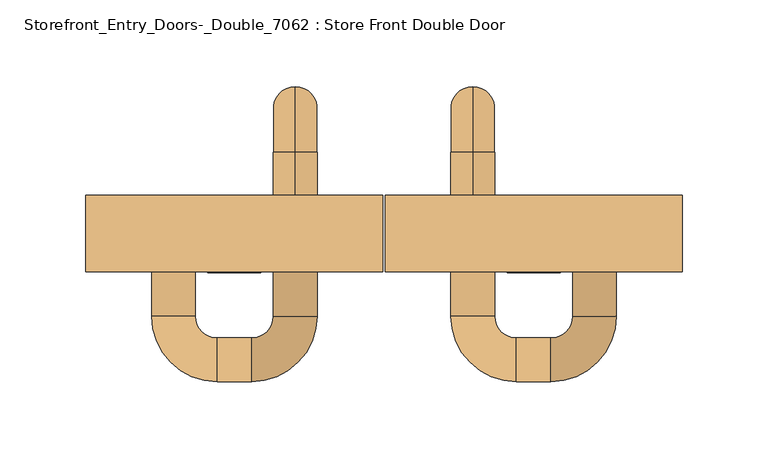
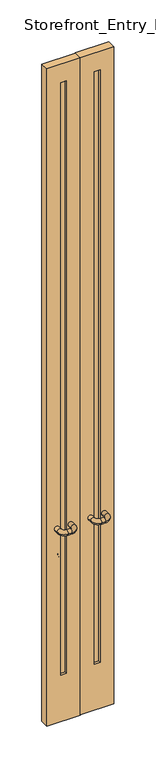
"""IFC4 building model written with IfcOpenShell, lengths in millimetres: door geometry, Storefront_Entry_Doors-_Double_7062 : Store Front Double Door."""

import ifcopenshell
import ifcopenshell.guid

model = None  # the IFC model being written
_history = None  # IfcOwnerHistory: only IFC2X3 demands one
_inside = {}  # id of a spatial element -> (the spatial element, [elements in it])
_under = {}  # id of a project, library or spatial element -> (it, [spatial elements below it])
_declared = {}  # id of a project -> (the project, [libraries it declares])
_typed = {}  # id of a type object -> (the type object, [elements of that type])
_made_of = {}  # id of a material, layer set ... -> (it, [elements and type objects made of it])


def new_model(schema):
    """Start an empty IFC model of exactly this schema.

    Asked for "IFC4X3", IfcOpenShell would pick the latest addendum, in which some entities
    have other attributes; the version numbers below select the first issue.
    IFC2X3 requires an IfcOwnerHistory on every rooted entity: one is made here for all.
    """
    global model, _history
    if schema == "IFC4X3":
        model = ifcopenshell.file(schema_version=(4, 3, 0, 0))
    else:
        model = ifcopenshell.file(schema=schema)
    _inside.clear()
    _under.clear()
    _declared.clear()
    _typed.clear()
    _made_of.clear()
    _history = None
    if model.schema == "IFC2X3":
        org = make("IfcOrganization", Name="unknown")
        user = make(
            "IfcPersonAndOrganization",
            ThePerson=make("IfcPerson", FamilyName="unknown"),
            TheOrganization=org,
        )
        app = make(
            "IfcApplication",
            ApplicationDeveloper=org,
            Version="unknown",
            ApplicationFullName="unknown",
            ApplicationIdentifier="unknown",
        )
        _history = make(
            "IfcOwnerHistory",
            OwningUser=user,
            OwningApplication=app,
            ChangeAction="ADDED",
            CreationDate=0,
        )
    return model


def make(cls, **values):
    """One entity of the class cls with the attributes given. An attribute that is None is left unset."""
    return model.create_entity(
        cls, **{name: value for name, value in values.items() if value is not None}
    )


def rooted(cls, **values):
    """An entity with a GlobalId (a new one), such as an element, a storey or a relation."""
    return make(cls, GlobalId=ifcopenshell.guid.new(), OwnerHistory=_history, **values)


def si_unit(unit_type, name, prefix=None):
    """IfcSIUnit, for example si_unit("LENGTHUNIT", "METRE", prefix="MILLI")."""
    return make("IfcSIUnit", UnitType=unit_type, Prefix=prefix, Name=name)


def assignment(units):
    """IfcUnitAssignment: the units of a project."""
    return None if units is None else make("IfcUnitAssignment", Units=units)


def point(xyz):
    """IfcCartesianPoint."""
    return None if xyz is None else make("IfcCartesianPoint", Coordinates=xyz)


def direction(xyz):
    """IfcDirection."""
    return None if xyz is None else make("IfcDirection", DirectionRatios=xyz)


def frame(location, z_axis=None, x_axis=None):
    """IfcAxis2Placement3D, a coordinate frame: its origin and axes. An axis left out is left unset."""
    return make(
        "IfcAxis2Placement3D",
        Location=point(location),
        Axis=direction(z_axis),
        RefDirection=direction(x_axis),
    )


def origin():
    """The frame at (0, 0, 0) with its axes left unset."""
    return frame((0.0, 0.0, 0.0))


def place(relative_to, where):
    """IfcLocalPlacement: puts the frame where relative to a parent placement (None: the world)."""
    return make(
        "IfcLocalPlacement", PlacementRelTo=relative_to, RelativePlacement=where
    )


def context(
    kind, dimensions, precision=None, world=None, true_north=None, identifier=None
):
    """IfcGeometricRepresentationContext, for example the 3D "Model" context."""
    return make(
        "IfcGeometricRepresentationContext",
        ContextIdentifier=identifier,
        ContextType=kind,
        CoordinateSpaceDimension=dimensions,
        Precision=precision,
        WorldCoordinateSystem=world,
        TrueNorth=true_north,
    )


def project(units=None, contexts=None):
    """IfcProject with its units and contexts."""
    return rooted(
        "IfcProject",
        Name="project",
        RepresentationContexts=contexts,
        UnitsInContext=assignment(units),
    )


def spatial(cls, under=None, at=None, **own):
    """A site, building, storey or space (cls), placed at a placement, below another one or the project."""
    s = rooted(cls, ObjectPlacement=at, **own)
    if under is not None:
        _under.setdefault(under.id(), (under, []))[1].append(s)
    return s


def polyline(points):
    """IfcPolyline through the points."""
    return make("IfcPolyline", Points=[point(p) for p in points])


def circle_curve(where, radius):
    """IfcCircle in the frame where."""
    return make("IfcCircle", Position=where, Radius=radius)


def ellipse_curve(where, semi_axis1, semi_axis2):
    """IfcEllipse in the frame where."""
    return make(
        "IfcEllipse", Position=where, SemiAxis1=semi_axis1, SemiAxis2=semi_axis2
    )


def trimmed(basis, trim1, trim2, sense, master):
    """IfcTrimmedCurve: the piece of a basis curve between two trims."""
    return make(
        "IfcTrimmedCurve",
        BasisCurve=basis,
        Trim1=trim1,
        Trim2=trim2,
        SenseAgreement=sense,
        MasterRepresentation=master,
    )


def outline(outer, holes=None, kind="AREA"):
    """IfcArbitraryClosedProfileDef: a profile drawn as a closed curve; with holes, ...WithVoids."""
    if holes is None:
        return make("IfcArbitraryClosedProfileDef", ProfileType=kind, OuterCurve=outer)
    return make(
        "IfcArbitraryProfileDefWithVoids",
        ProfileType=kind,
        OuterCurve=outer,
        InnerCurves=holes,
    )


def extrude(swept, where, along, depth):
    """IfcExtrudedAreaSolid: the profile swept, set in the frame where, extruded along a direction by depth."""
    return make(
        "IfcExtrudedAreaSolid",
        SweptArea=swept,
        Position=where,
        ExtrudedDirection=direction(along),
        Depth=depth,
    )


def shape(context_of_items, identifier, shape_type, items):
    """IfcShapeRepresentation: the items that make up one representation, for example the "Body"."""
    return make(
        "IfcShapeRepresentation",
        ContextOfItems=context_of_items,
        RepresentationIdentifier=identifier,
        RepresentationType=shape_type,
        Items=items,
    )


def source(mapping_origin, context_of_items, identifier, shape_type, items):
    """IfcRepresentationMap: a shape defined once, which mapped items show again and again."""
    return make(
        "IfcRepresentationMap",
        MappingOrigin=mapping_origin,
        MappedRepresentation=shape(context_of_items, identifier, shape_type, items),
    )


def transform(
    local_origin,
    x_axis=None,
    y_axis=None,
    z_axis=None,
    scale=None,
    scale2=None,
    scale3=None,
    uniform=True,
):
    """IfcCartesianTransformationOperator3D, or its non-uniform kind. x_axis, y_axis, z_axis: its Axis1, 2, 3."""
    if uniform:
        return make(
            "IfcCartesianTransformationOperator3D",
            Axis1=direction(x_axis),
            Axis2=direction(y_axis),
            LocalOrigin=point(local_origin),
            Scale=scale,
            Axis3=direction(z_axis),
        )
    return make(
        "IfcCartesianTransformationOperator3DnonUniform",
        Axis1=direction(x_axis),
        Axis2=direction(y_axis),
        LocalOrigin=point(local_origin),
        Scale=scale,
        Axis3=direction(z_axis),
        Scale2=scale2,
        Scale3=scale3,
    )


def mapped(mapping_source, mapping_target):
    """IfcMappedItem: shows the shape of a source again, moved by a transform."""
    return make(
        "IfcMappedItem", MappingSource=mapping_source, MappingTarget=mapping_target
    )


def made_of(thing, what):
    """Note that an element or type object is made of a material, layer set ...; save() writes the relation."""
    if what is not None:
        _made_of.setdefault(what.id(), (what, []))[1].append(thing)
    return thing


def element(
    cls,
    number,
    at=None,
    inside=None,
    cuts=None,
    type_object=None,
    material=None,
    context=None,
    identifier="Body",
    shape_type=None,
    held_by="IfcProductDefinitionShape",
    body=None,
    shapes=None,
    **own,
):
    """One element of the class cls, such as IfcWall. Its Tag is "e" and its number.

    at: its placement. inside: the storey or other place that contains it. cuts: it is an
    opening in that element (IfcRelVoidsElement). A single representation is given by context,
    identifier, shape_type and body (its items); several are given by shapes. held_by: the class
    of the entity that holds the representations. save() writes the other relations.
    """
    e = rooted(cls, Tag="e%d" % number, ObjectPlacement=at, **own)
    if body is not None:
        shapes = [shape(context, identifier, shape_type, body)]
    if shapes is not None:
        e.Representation = make(held_by, Representations=shapes)
    if inside is not None:
        _inside.setdefault(inside.id(), (inside, []))[1].append(e)
    if cuts is not None:
        rooted(
            "IfcRelVoidsElement", RelatingBuildingElement=cuts, RelatedOpeningElement=e
        )
    if type_object is not None:
        _typed.setdefault(type_object.id(), (type_object, []))[1].append(e)
    return made_of(e, material)


def aggregate(whole, parts):
    """IfcRelAggregates: a whole, such as a stair, and the parts it consists of."""
    return rooted("IfcRelAggregates", RelatingObject=whole, RelatedObjects=parts)


def save(model, path):
    """Write the relations noted so far, then the file.

    IfcRelAggregates (storeys below a building ...), IfcRelContainedInSpatialStructure (elements
    in a storey), IfcRelDefinesByType, IfcRelAssociatesMaterial and IfcRelDeclares: one each for
    every whole, place, type object, material and project.
    """
    for whole, parts in _under.values():
        aggregate(whole, parts)
    for where, things in _inside.values():
        rooted(
            "IfcRelContainedInSpatialStructure",
            RelatedElements=things,
            RelatingStructure=where,
        )
    for kind, things in _typed.values():
        rooted("IfcRelDefinesByType", RelatedObjects=things, RelatingType=kind)
    for what, things in _made_of.values():
        rooted("IfcRelAssociatesMaterial", RelatedObjects=things, RelatingMaterial=what)
    for by, libraries in _declared.values():
        rooted("IfcRelDeclares", RelatingContext=by, RelatedDefinitions=libraries)
    model.write(path)


def plane_surface(at):
    """IfcPlane: the flat surface through the origin of the frame at, square to its z axis."""
    return make("IfcPlane", Position=at)


def cylinder_surface(at, radius):
    """IfcCylindricalSurface: all points at the distance radius from the z axis of the frame at."""
    return make("IfcCylindricalSurface", Position=at, Radius=radius)


def revolved_surface(curve, axis_point, axis_direction):
    """IfcSurfaceOfRevolution: the curve turned about the line through axis_point along axis_direction."""
    return make(
        "IfcSurfaceOfRevolution",
        SweptCurve=make("IfcArbitraryOpenProfileDef", ProfileType="CURVE", Curve=curve),
        AxisPosition=make("IfcAxis1Placement", Location=point(axis_point), Axis=direction(axis_direction)),
    )


def advanced_brep(points, edges, surfaces, faces):
    """IfcAdvancedBrep: a solid bounded by faces that lie on surfaces and meet in shared edges.

    An edge is (start, end): straight between two places in points (the first is 0);
    or (start, end, curve); or (start, end, curve, False) where it runs against its curve.
    A face is (place in surfaces, loops), or (place, loops, False) where it looks against
    its surface's normal. A loop lists edges by number (the first is 1), with a minus sign
    where the edge is run from its end to its start. The first loop is the outer one.
    """
    corners = [point(p) for p in points]
    vertices = [make("IfcVertexPoint", VertexGeometry=c) for c in corners]
    made = []
    for start, end, *more in edges:
        made.append(
            make(
                "IfcEdgeCurve",
                EdgeStart=vertices[start],
                EdgeEnd=vertices[end],
                EdgeGeometry=more[0] if more else make("IfcPolyline", Points=[corners[start], corners[end]]),
                SameSense=more[1] if len(more) > 1 else True,
            )
        )
    hull = []
    for where, loops, *sense in faces:
        bounds = []
        for j, loop in enumerate(loops):
            ring = [make("IfcOrientedEdge", EdgeElement=made[abs(k) - 1], Orientation=k > 0) for k in loop]
            bounds.append(
                make(
                    "IfcFaceOuterBound" if j == 0 else "IfcFaceBound",
                    Bound=make("IfcEdgeLoop", EdgeList=ring),
                    Orientation=True,
                )
            )
        hull.append(make("IfcAdvancedFace", Bounds=bounds, FaceSurface=surfaces[where], SameSense=sense[0] if sense else True))
    return make("IfcAdvancedBrep", Outer=make("IfcClosedShell", CfsFaces=hull))


def storefront_entry_doors_double_7062_store_front_double_door_a2ad6f36(model_context):
    return source(origin(), model_context, "Body", "SolidModel", [
        advanced_brep(
        [(51.59375, 50.8, 1079.5), (51.59375, 50.8, 1054.1), (51.59375, 76.2, 1079.5), (51.59375, 76.2, 1054.1), (51.59375, 88.9, 1041.4), (51.59375, 114.3, 1041.4), (51.59375, 114.3, 863.6), (51.59375, 88.9, 863.6), (51.59375, 76.2, 850.9), (51.59375, 76.2, 825.5), (51.59375, 50.8, 825.5), (51.59375, 50.8, 850.9)],
        [
            (0, 1, circle_curve(frame((51.59375, 50.8, 1066.8), z_axis=(0.0, -1.0, 0.0), x_axis=(0.0, 0.0, -1.0)), 12.7)),
            (1, 0, circle_curve(frame((51.59375, 50.8, 1066.8), z_axis=(0.0, -1.0, 0.0), x_axis=(0.0, 0.0, -1.0)), 12.7)),
            (0, 2),
            (2, 3, circle_curve(frame((51.59375, 76.2, 1066.8), z_axis=(0.0, -1.0, 0.0), x_axis=(0.0, 0.0, -1.0)), 12.7)),
            (3, 1),
            (3, 2, circle_curve(frame((51.59375, 76.2, 1066.8), z_axis=(0.0, -1.0, 0.0), x_axis=(0.0, 0.0, -1.0)), 12.7)),
            (4, 3, circle_curve(frame((51.59375, 76.2, 1041.4), z_axis=(1.0, 0.0, 0.0), x_axis=(0.0, 0.0, 1.0)), 12.7)),
            (2, 5, circle_curve(frame((51.59375, 76.2, 1041.4), z_axis=(-1.0, 0.0, 0.0), x_axis=(0.0, 0.0, 1.0)), 38.1)),
            (5, 4, circle_curve(frame((51.59375, 101.6, 1041.4), z_axis=(0.0, 0.0, 1.0), x_axis=(0.0, -1.0, 0.0)), 12.7)),
            (4, 5, circle_curve(frame((51.59375, 101.6, 1041.4), z_axis=(0.0, 0.0, 1.0), x_axis=(0.0, -1.0, 0.0)), 12.7)),
            (5, 6),
            (6, 7, circle_curve(frame((51.59375, 101.6, 863.6), z_axis=(0.0, 0.0, 1.0), x_axis=(0.0, -1.0, 0.0)), 12.7)),
            (7, 4),
            (7, 6, circle_curve(frame((51.59375, 101.6, 863.6), z_axis=(0.0, 0.0, 1.0), x_axis=(0.0, -1.0, 0.0)), 12.7)),
            (8, 7, circle_curve(frame((51.59375, 76.2, 863.6), z_axis=(1.0, 0.0, 0.0), x_axis=(0.0, 1.0, 0.0)), 12.7)),
            (6, 9, circle_curve(frame((51.59375, 76.2, 863.6), z_axis=(-1.0, 0.0, 0.0), x_axis=(0.0, 1.0, 0.0)), 38.1)),
            (9, 8, circle_curve(frame((51.59375, 76.2, 838.2), z_axis=(0.0, 1.0, 0.0), x_axis=(0.0, 0.0, 1.0)), 12.7)),
            (8, 9, circle_curve(frame((51.59375, 76.2, 838.2), z_axis=(0.0, 1.0, 0.0), x_axis=(0.0, 0.0, 1.0)), 12.7)),
            (10, 11, circle_curve(frame((51.59375, 50.8, 838.2), z_axis=(0.0, -1.0, 0.0), x_axis=(0.0, 0.0, 1.0)), 12.7)),
            (11, 10, circle_curve(frame((51.59375, 50.8, 838.2), z_axis=(0.0, -1.0, 0.0), x_axis=(0.0, 0.0, 1.0)), 12.7)),
            (9, 10),
            (11, 8),
        ],
        [
            plane_surface(frame((51.59375, 50.8, 1066.8), z_axis=(0.0, -1.0, 0.0), x_axis=(-1.0, 0.0, 0.0))),
            cylinder_surface(frame((51.59375, 50.8, 1066.8), z_axis=(0.0, -1.0, 0.0), x_axis=(0.0, 0.0, -1.0)), 12.7),
            revolved_surface(trimmed(ellipse_curve(frame((51.59375, 76.2, 1066.8), z_axis=(0.0, -1.0, 0.0), x_axis=(0.0, 0.0, -1.0)), 12.7, 12.7), [point((51.59375, 76.2, 1079.5))], [point((51.59375, 76.2, 1054.1))], True, "CARTESIAN"), (51.59375, 76.2, 1041.4), (-1.0, 0.0, 0.0)),
            revolved_surface(trimmed(ellipse_curve(frame((51.59375, 76.2, 1066.8), z_axis=(0.0, -1.0, 0.0), x_axis=(0.0, 0.0, -1.0)), 12.7, 12.7), [point((51.59375, 76.2, 1054.1))], [point((51.59375, 76.2, 1079.5))], True, "CARTESIAN"), (51.59375, 76.2, 1041.4), (-1.0, 0.0, 0.0)),
            cylinder_surface(frame((51.59375, 101.6, 1041.4), z_axis=(0.0, 0.0, 1.0), x_axis=(0.0, -1.0, 0.0)), 12.7),
            revolved_surface(trimmed(ellipse_curve(frame((51.59375, 101.6, 863.6), z_axis=(0.0, 0.0, 1.0), x_axis=(0.0, -1.0, 0.0)), 12.7, 12.7), [point((51.59375, 114.3, 863.6))], [point((51.59375, 88.9, 863.6))], True, "CARTESIAN"), (51.59375, 76.2, 863.6), (-1.0, 0.0, 0.0)),
            revolved_surface(trimmed(ellipse_curve(frame((51.59375, 101.6, 863.6), z_axis=(0.0, 0.0, 1.0), x_axis=(0.0, -1.0, 0.0)), 12.7, 12.7), [point((51.59375, 88.9, 863.6))], [point((51.59375, 114.3, 863.6))], True, "CARTESIAN"), (51.59375, 76.2, 863.6), (-1.0, 0.0, 0.0)),
            plane_surface(frame((51.59375, 50.8, 838.2), z_axis=(0.0, -1.0, 0.0), x_axis=(-1.0, 0.0, 0.0))),
            cylinder_surface(frame((51.59375, 76.2, 838.2), z_axis=(0.0, 1.0, 0.0), x_axis=(0.0, 0.0, 1.0)), 12.7),
        ],
        [
            (0, [[1, 2]]),
            (1, [[-1, 3, 4, 5]]),
            (1, [[-2, -5, 6, -3]]),
            (2, [[7, -4, 8, 9]]),
            (3, [[-8, -6, -7, 10]]),
            (4, [[-9, 11, 12, 13]]),
            (4, [[-10, -13, 14, -11]]),
            (5, [[15, -12, 16, 17]]),
            (6, [[-16, -14, -15, 18]]),
            (7, [[19, 20]]),
            (8, [[-17, 21, -20, 22]]),
            (8, [[-18, -22, -19, -21]]),
        ],
    ),
        advanced_brep(
        [(109.7642857, 6.35, 1066.8), (135.1642857, 6.35, 1066.8), (109.7642857, -19.05, 1066.8), (135.1642857, -19.05, 1066.8), (97.0642857, -57.15, 1066.8), (97.0642857, -31.75, 1066.8), (76.99375, -31.75, 1066.8), (76.99375, -57.15, 1066.8), (38.89375, -19.05, 1066.8), (64.29375, -19.05, 1066.8), (64.29375, 6.35, 1066.8), (38.89375, 6.35, 1066.8)],
        [
            (0, 1, circle_curve(frame((122.4642857, 6.35, 1066.8), z_axis=(0.0, 1.0, 0.0), x_axis=(1.0, 0.0, 0.0)), 12.7)),
            (1, 0, circle_curve(frame((122.4642857, 6.35, 1066.8), z_axis=(0.0, 1.0, 0.0), x_axis=(1.0, 0.0, 0.0)), 12.7)),
            (0, 2),
            (2, 3, circle_curve(frame((122.4642857, -19.05, 1066.8), z_axis=(0.0, 1.0, 0.0), x_axis=(1.0, 0.0, 0.0)), 12.7)),
            (3, 1),
            (3, 2, circle_curve(frame((122.4642857, -19.05, 1066.8), z_axis=(0.0, 1.0, 0.0), x_axis=(1.0, 0.0, 0.0)), 12.7)),
            (4, 3, circle_curve(frame((97.0642857, -19.05, 1066.8), z_axis=(0.0, 0.0, 1.0), x_axis=(1.0, 0.0, 0.0)), 38.1)),
            (2, 5, circle_curve(frame((97.0642857, -19.05, 1066.8), z_axis=(0.0, 0.0, -1.0), x_axis=(1.0, 0.0, 0.0)), 12.7)),
            (5, 4, circle_curve(frame((97.0642857, -44.45, 1066.8), z_axis=(1.0, 0.0, 0.0), x_axis=(0.0, -1.0, 0.0)), 12.7)),
            (4, 5, circle_curve(frame((97.0642857, -44.45, 1066.8), z_axis=(1.0, 0.0, 0.0), x_axis=(0.0, -1.0, 0.0)), 12.7)),
            (5, 6),
            (6, 7, circle_curve(frame((76.99375, -44.45, 1066.8), z_axis=(1.0, 0.0, 0.0), x_axis=(0.0, -1.0, 0.0)), 12.7)),
            (7, 4),
            (7, 6, circle_curve(frame((76.99375, -44.45, 1066.8), z_axis=(1.0, 0.0, 0.0), x_axis=(0.0, -1.0, 0.0)), 12.7)),
            (8, 7, circle_curve(frame((76.99375, -19.05, 1066.8), z_axis=(0.0, 0.0, 1.0), x_axis=(0.0, -1.0, 0.0)), 38.1)),
            (6, 9, circle_curve(frame((76.99375, -19.05, 1066.8), z_axis=(0.0, 0.0, -1.0), x_axis=(0.0, -1.0, 0.0)), 12.7)),
            (9, 8, circle_curve(frame((51.59375, -19.05, 1066.8), z_axis=(0.0, -1.0, 0.0), x_axis=(-1.0, 0.0, 0.0)), 12.7)),
            (8, 9, circle_curve(frame((51.59375, -19.05, 1066.8), z_axis=(0.0, -1.0, 0.0), x_axis=(-1.0, 0.0, 0.0)), 12.7)),
            (10, 11, circle_curve(frame((51.59375, 6.35, 1066.8), z_axis=(0.0, 1.0, 0.0), x_axis=(-1.0, 0.0, 0.0)), 12.7)),
            (11, 10, circle_curve(frame((51.59375, 6.35, 1066.8), z_axis=(0.0, 1.0, 0.0), x_axis=(-1.0, 0.0, 0.0)), 12.7)),
            (9, 10),
            (11, 8),
        ],
        [
            plane_surface(frame((122.4642857, 6.35, 1066.8), z_axis=(0.0, 1.0, 0.0), x_axis=(0.0, 0.0, 1.0))),
            cylinder_surface(frame((122.4642857, 6.35, 1066.8), z_axis=(0.0, 1.0, 0.0), x_axis=(1.0, 0.0, 0.0)), 12.7),
            revolved_surface(trimmed(ellipse_curve(frame((122.4642857, -19.05, 1066.8), z_axis=(0.0, 1.0, 0.0), x_axis=(1.0, 0.0, 0.0)), 12.7, 12.7), [point((109.7642857, -19.05, 1066.8))], [point((135.1642857, -19.05, 1066.8))], True, "CARTESIAN"), (97.0642857, -19.05, 1066.8), (0.0, 0.0, -1.0)),
            revolved_surface(trimmed(ellipse_curve(frame((122.4642857, -19.05, 1066.8), z_axis=(0.0, 1.0, 0.0), x_axis=(1.0, 0.0, 0.0)), 12.7, 12.7), [point((135.1642857, -19.05, 1066.8))], [point((109.7642857, -19.05, 1066.8))], True, "CARTESIAN"), (97.0642857, -19.05, 1066.8), (0.0, 0.0, -1.0)),
            cylinder_surface(frame((97.0642857, -44.45, 1066.8), z_axis=(1.0, 0.0, 0.0), x_axis=(0.0, -1.0, 0.0)), 12.7),
            revolved_surface(trimmed(ellipse_curve(frame((76.99375, -44.45, 1066.8), z_axis=(1.0, 0.0, 0.0), x_axis=(0.0, -1.0, 0.0)), 12.7, 12.7), [point((76.99375, -31.75, 1066.8))], [point((76.99375, -57.15, 1066.8))], True, "CARTESIAN"), (76.99375, -19.05, 1066.8), (0.0, 0.0, -1.0)),
            revolved_surface(trimmed(ellipse_curve(frame((76.99375, -44.45, 1066.8), z_axis=(1.0, 0.0, 0.0), x_axis=(0.0, -1.0, 0.0)), 12.7, 12.7), [point((76.99375, -57.15, 1066.8))], [point((76.99375, -31.75, 1066.8))], True, "CARTESIAN"), (76.99375, -19.05, 1066.8), (0.0, 0.0, -1.0)),
            plane_surface(frame((51.59375, 6.35, 1066.8), z_axis=(0.0, 1.0, 0.0), x_axis=(0.0, 0.0, 1.0))),
            cylinder_surface(frame((51.59375, -19.05, 1066.8), z_axis=(0.0, -1.0, 0.0), x_axis=(-1.0, 0.0, 0.0)), 12.7),
        ],
        [
            (0, [[1, 2]]),
            (1, [[-1, 3, 4, 5]]),
            (1, [[-2, -5, 6, -3]]),
            (2, [[7, -4, 8, 9]]),
            (3, [[-8, -6, -7, 10]]),
            (4, [[-9, 11, 12, 13]]),
            (4, [[-10, -13, 14, -11]]),
            (5, [[15, -12, 16, 17]]),
            (6, [[-16, -14, -15, 18]]),
            (7, [[19, 20]]),
            (8, [[-17, 21, -20, 22]]),
            (8, [[-18, -22, -19, -21]]),
        ],
    ),
        advanced_brep(
        [(-51.59375, 50.8, 1054.1), (-51.59375, 50.8, 1079.5), (-51.59375, 76.2, 1054.1), (-51.59375, 76.2, 1079.5), (-51.59375, 114.3, 1041.4), (-51.59375, 88.9, 1041.4), (-51.59375, 88.9, 863.6), (-51.59375, 114.3, 863.6), (-51.59375, 76.2, 825.5), (-51.59375, 76.2, 850.9), (-51.59375, 50.8, 850.9), (-51.59375, 50.8, 825.5)],
        [
            (0, 1, circle_curve(frame((-51.59375, 50.8, 1066.8), z_axis=(0.0, -1.0, 0.0), x_axis=(0.0, 0.0, 1.0)), 12.7)),
            (1, 0, circle_curve(frame((-51.59375, 50.8, 1066.8), z_axis=(0.0, -1.0, 0.0), x_axis=(0.0, 0.0, 1.0)), 12.7)),
            (0, 2),
            (2, 3, circle_curve(frame((-51.59375, 76.2, 1066.8), z_axis=(0.0, -1.0, 0.0), x_axis=(0.0, 0.0, 1.0)), 12.7)),
            (3, 1),
            (3, 2, circle_curve(frame((-51.59375, 76.2, 1066.8), z_axis=(0.0, -1.0, 0.0), x_axis=(0.0, 0.0, 1.0)), 12.7)),
            (4, 3, circle_curve(frame((-51.59375, 76.2, 1041.4), z_axis=(1.0, 0.0, 0.0), x_axis=(0.0, 0.0, 1.0)), 38.1)),
            (2, 5, circle_curve(frame((-51.59375, 76.2, 1041.4), z_axis=(-1.0, 0.0, 0.0), x_axis=(0.0, 0.0, 1.0)), 12.7)),
            (5, 4, circle_curve(frame((-51.59375, 101.6, 1041.4), z_axis=(0.0, 0.0, 1.0), x_axis=(0.0, 1.0, 0.0)), 12.7)),
            (4, 5, circle_curve(frame((-51.59375, 101.6, 1041.4), z_axis=(0.0, 0.0, 1.0), x_axis=(0.0, 1.0, 0.0)), 12.7)),
            (5, 6),
            (6, 7, circle_curve(frame((-51.59375, 101.6, 863.6), z_axis=(0.0, 0.0, 1.0), x_axis=(0.0, 1.0, 0.0)), 12.7)),
            (7, 4),
            (7, 6, circle_curve(frame((-51.59375, 101.6, 863.6), z_axis=(0.0, 0.0, 1.0), x_axis=(0.0, 1.0, 0.0)), 12.7)),
            (8, 7, circle_curve(frame((-51.59375, 76.2, 863.6), z_axis=(1.0, 0.0, 0.0), x_axis=(0.0, 1.0, 0.0)), 38.1)),
            (6, 9, circle_curve(frame((-51.59375, 76.2, 863.6), z_axis=(-1.0, 0.0, 0.0), x_axis=(0.0, 1.0, 0.0)), 12.7)),
            (9, 8, circle_curve(frame((-51.59375, 76.2, 838.2), z_axis=(0.0, 1.0, 0.0), x_axis=(0.0, 0.0, -1.0)), 12.7)),
            (8, 9, circle_curve(frame((-51.59375, 76.2, 838.2), z_axis=(0.0, 1.0, 0.0), x_axis=(0.0, 0.0, -1.0)), 12.7)),
            (10, 11, circle_curve(frame((-51.59375, 50.8, 838.2), z_axis=(0.0, -1.0, 0.0), x_axis=(0.0, 0.0, -1.0)), 12.7)),
            (11, 10, circle_curve(frame((-51.59375, 50.8, 838.2), z_axis=(0.0, -1.0, 0.0), x_axis=(0.0, 0.0, -1.0)), 12.7)),
            (9, 10),
            (11, 8),
        ],
        [
            plane_surface(frame((-51.59375, 50.8, 1066.8), z_axis=(0.0, -1.0, 0.0), x_axis=(1.0, 0.0, 0.0))),
            cylinder_surface(frame((-51.59375, 50.8, 1066.8), z_axis=(0.0, -1.0, 0.0), x_axis=(0.0, 0.0, 1.0)), 12.7),
            revolved_surface(trimmed(ellipse_curve(frame((-51.59375, 76.2, 1066.8), z_axis=(0.0, -1.0, 0.0), x_axis=(0.0, 0.0, 1.0)), 12.7, 12.7), [point((-51.59375, 76.2, 1054.1))], [point((-51.59375, 76.2, 1079.5))], True, "CARTESIAN"), (-51.59375, 76.2, 1041.4), (-1.0, 0.0, 0.0)),
            revolved_surface(trimmed(ellipse_curve(frame((-51.59375, 76.2, 1066.8), z_axis=(0.0, -1.0, 0.0), x_axis=(0.0, 0.0, 1.0)), 12.7, 12.7), [point((-51.59375, 76.2, 1079.5))], [point((-51.59375, 76.2, 1054.1))], True, "CARTESIAN"), (-51.59375, 76.2, 1041.4), (-1.0, 0.0, 0.0)),
            cylinder_surface(frame((-51.59375, 101.6, 1041.4), z_axis=(0.0, 0.0, 1.0), x_axis=(0.0, 1.0, 0.0)), 12.7),
            revolved_surface(trimmed(ellipse_curve(frame((-51.59375, 101.6, 863.6), z_axis=(0.0, 0.0, 1.0), x_axis=(0.0, 1.0, 0.0)), 12.7, 12.7), [point((-51.59375, 88.9, 863.6))], [point((-51.59375, 114.3, 863.6))], True, "CARTESIAN"), (-51.59375, 76.2, 863.6), (-1.0, 0.0, 0.0)),
            revolved_surface(trimmed(ellipse_curve(frame((-51.59375, 101.6, 863.6), z_axis=(0.0, 0.0, 1.0), x_axis=(0.0, 1.0, 0.0)), 12.7, 12.7), [point((-51.59375, 114.3, 863.6))], [point((-51.59375, 88.9, 863.6))], True, "CARTESIAN"), (-51.59375, 76.2, 863.6), (-1.0, 0.0, 0.0)),
            plane_surface(frame((-51.59375, 50.8, 838.2), z_axis=(0.0, -1.0, 0.0), x_axis=(1.0, 0.0, 0.0))),
            cylinder_surface(frame((-51.59375, 76.2, 838.2), z_axis=(0.0, 1.0, 0.0), x_axis=(0.0, 0.0, -1.0)), 12.7),
        ],
        [
            (0, [[1, 2]]),
            (1, [[-1, 3, 4, 5]]),
            (1, [[-2, -5, 6, -3]]),
            (2, [[7, -4, 8, 9]]),
            (3, [[-8, -6, -7, 10]]),
            (4, [[-9, 11, 12, 13]]),
            (4, [[-10, -13, 14, -11]]),
            (5, [[15, -12, 16, 17]]),
            (6, [[-16, -14, -15, 18]]),
            (7, [[19, 20]]),
            (8, [[-17, 21, -20, 22]]),
            (8, [[-18, -22, -19, -21]]),
        ],
    ),
        advanced_brep(
        [(-64.29375, 6.35, 1066.8), (-38.89375, 6.35, 1066.8), (-64.29375, -19.05, 1066.8), (-38.89375, -19.05, 1066.8), (-76.99375, -57.15, 1066.8), (-76.99375, -31.75, 1066.8), (-97.0642857, -31.75, 1066.8), (-97.0642857, -57.15, 1066.8), (-135.1642857, -19.05, 1066.8), (-109.7642857, -19.05, 1066.8), (-109.7642857, 6.35, 1066.8), (-135.1642857, 6.35, 1066.8)],
        [
            (0, 1, circle_curve(frame((-51.59375, 6.35, 1066.8), z_axis=(0.0, 1.0, 0.0), x_axis=(1.0, 0.0, 0.0)), 12.7)),
            (1, 0, circle_curve(frame((-51.59375, 6.35, 1066.8), z_axis=(0.0, 1.0, 0.0), x_axis=(1.0, 0.0, 0.0)), 12.7)),
            (0, 2),
            (2, 3, circle_curve(frame((-51.59375, -19.05, 1066.8), z_axis=(0.0, 1.0, 0.0), x_axis=(1.0, 0.0, 0.0)), 12.7)),
            (3, 1),
            (3, 2, circle_curve(frame((-51.59375, -19.05, 1066.8), z_axis=(0.0, 1.0, 0.0), x_axis=(1.0, 0.0, 0.0)), 12.7)),
            (4, 3, circle_curve(frame((-76.99375, -19.05, 1066.8), z_axis=(0.0, 0.0, 1.0), x_axis=(1.0, 0.0, 0.0)), 38.1)),
            (2, 5, circle_curve(frame((-76.99375, -19.05, 1066.8), z_axis=(0.0, 0.0, -1.0), x_axis=(1.0, 0.0, 0.0)), 12.7)),
            (5, 4, circle_curve(frame((-76.99375, -44.45, 1066.8), z_axis=(1.0, 0.0, 0.0), x_axis=(0.0, -1.0, 0.0)), 12.7)),
            (4, 5, circle_curve(frame((-76.99375, -44.45, 1066.8), z_axis=(1.0, 0.0, 0.0), x_axis=(0.0, -1.0, 0.0)), 12.7)),
            (5, 6),
            (6, 7, circle_curve(frame((-97.0642857, -44.45, 1066.8), z_axis=(1.0, 0.0, 0.0), x_axis=(0.0, -1.0, 0.0)), 12.7)),
            (7, 4),
            (7, 6, circle_curve(frame((-97.0642857, -44.45, 1066.8), z_axis=(1.0, 0.0, 0.0), x_axis=(0.0, -1.0, 0.0)), 12.7)),
            (8, 7, circle_curve(frame((-97.0642857, -19.05, 1066.8), z_axis=(0.0, 0.0, 1.0), x_axis=(0.0, -1.0, 0.0)), 38.1)),
            (6, 9, circle_curve(frame((-97.0642857, -19.05, 1066.8), z_axis=(0.0, 0.0, -1.0), x_axis=(0.0, -1.0, 0.0)), 12.7)),
            (9, 8, circle_curve(frame((-122.4642857, -19.05, 1066.8), z_axis=(0.0, -1.0, 0.0), x_axis=(-1.0, 0.0, 0.0)), 12.7)),
            (8, 9, circle_curve(frame((-122.4642857, -19.05, 1066.8), z_axis=(0.0, -1.0, 0.0), x_axis=(-1.0, 0.0, 0.0)), 12.7)),
            (10, 11, circle_curve(frame((-122.4642857, 6.35, 1066.8), z_axis=(0.0, 1.0, 0.0), x_axis=(-1.0, 0.0, 0.0)), 12.7)),
            (11, 10, circle_curve(frame((-122.4642857, 6.35, 1066.8), z_axis=(0.0, 1.0, 0.0), x_axis=(-1.0, 0.0, 0.0)), 12.7)),
            (9, 10),
            (11, 8),
        ],
        [
            plane_surface(frame((-51.59375, 6.35, 1066.8), z_axis=(0.0, 1.0, 0.0), x_axis=(0.0, 0.0, 1.0))),
            cylinder_surface(frame((-51.59375, 6.35, 1066.8), z_axis=(0.0, 1.0, 0.0), x_axis=(1.0, 0.0, 0.0)), 12.7),
            revolved_surface(trimmed(ellipse_curve(frame((-51.59375, -19.05, 1066.8), z_axis=(0.0, 1.0, 0.0), x_axis=(1.0, 0.0, 0.0)), 12.7, 12.7), [point((-64.29375, -19.05, 1066.8))], [point((-38.89375, -19.05, 1066.8))], True, "CARTESIAN"), (-76.99375, -19.05, 1066.8), (0.0, 0.0, -1.0)),
            revolved_surface(trimmed(ellipse_curve(frame((-51.59375, -19.05, 1066.8), z_axis=(0.0, 1.0, 0.0), x_axis=(1.0, 0.0, 0.0)), 12.7, 12.7), [point((-38.89375, -19.05, 1066.8))], [point((-64.29375, -19.05, 1066.8))], True, "CARTESIAN"), (-76.99375, -19.05, 1066.8), (0.0, 0.0, -1.0)),
            cylinder_surface(frame((-76.99375, -44.45, 1066.8), z_axis=(1.0, 0.0, 0.0), x_axis=(0.0, -1.0, 0.0)), 12.7),
            revolved_surface(trimmed(ellipse_curve(frame((-97.0642857, -44.45, 1066.8), z_axis=(1.0, 0.0, 0.0), x_axis=(0.0, -1.0, 0.0)), 12.7, 12.7), [point((-97.0642857, -31.75, 1066.8))], [point((-97.0642857, -57.15, 1066.8))], True, "CARTESIAN"), (-97.0642857, -19.05, 1066.8), (0.0, 0.0, -1.0)),
            revolved_surface(trimmed(ellipse_curve(frame((-97.0642857, -44.45, 1066.8), z_axis=(1.0, 0.0, 0.0), x_axis=(0.0, -1.0, 0.0)), 12.7, 12.7), [point((-97.0642857, -57.15, 1066.8))], [point((-97.0642857, -31.75, 1066.8))], True, "CARTESIAN"), (-97.0642857, -19.05, 1066.8), (0.0, 0.0, -1.0)),
            plane_surface(frame((-122.4642857, 6.35, 1066.8), z_axis=(0.0, 1.0, 0.0), x_axis=(0.0, 0.0, 1.0))),
            cylinder_surface(frame((-122.4642857, -19.05, 1066.8), z_axis=(0.0, -1.0, 0.0), x_axis=(-1.0, 0.0, 0.0)), 12.7),
        ],
        [
            (0, [[1, 2]]),
            (1, [[-1, 3, 4, 5]]),
            (1, [[-2, -5, 6, -3]]),
            (2, [[7, -4, 8, 9]]),
            (3, [[-8, -6, -7, 10]]),
            (4, [[-9, 11, 12, 13]]),
            (4, [[-10, -13, 14, -11]]),
            (5, [[15, -12, 16, 17]]),
            (6, [[-16, -14, -15, 18]]),
            (7, [[19, 20]]),
            (8, [[-17, 21, -20, 22]]),
            (8, [[-18, -22, -19, -21]]),
        ],
    ),
        extrude(outline(polyline([(102.39375, 19.05), (71.6642857, 19.05), (71.6642857, 38.1), (102.39375, 38.1), (102.39375, 19.05)])), frame((0.0, 0.0, 254.0), z_axis=(0.0, 0.0, 1.0), x_axis=(1.0, 0.0, 0.0)), (0.0, 0.0, 1.0), 3251.2),
        extrude(outline(polyline([(-71.6642857, 19.05), (-102.39375, 19.05), (-102.39375, 38.1), (-71.6642857, 38.1), (-71.6642857, 19.05)])), frame((0.0, 0.0, 254.0), z_axis=(0.0, 0.0, 1.0), x_axis=(1.0, 0.0, 0.0)), (0.0, 0.0, 1.0), 3251.2),
        extrude(outline(polyline([(3606.8, 0.79375), (0.0, 0.79375), (0.0, 173.2642857), (3606.8, 173.2642857), (3606.8, 0.79375)]), holes=[polyline([(3505.2, 102.39375), (254.0, 102.39375), (254.0, 71.6642857), (3505.2, 71.6642857), (3505.2, 102.39375)])]), frame((0.0, 6.35, 0.0), z_axis=(0.0, 1.0, 0.0), x_axis=(0.0, 0.0, 1.0)), (0.0, 0.0, 1.0), 44.45),
        extrude(outline(polyline([(3606.8, -0.79375), (3606.8, -173.2642857), (0.0, -173.2642857), (0.0, -0.79375), (3606.8, -0.79375)]), holes=[polyline([(3505.2, -71.6642857), (254.0, -71.6642857), (254.0, -102.39375), (3505.2, -102.39375), (3505.2, -71.6642857)])]), frame((0.0, 6.35, 0.0), z_axis=(0.0, 1.0, 0.0), x_axis=(0.0, 0.0, 1.0)), (0.0, 0.0, 1.0), 44.45),
    ])


if __name__ == "__main__":
    model = new_model("IFC4")
    model_context = context("Model", 3, world=origin())
    ifc_project = project(units=[si_unit("LENGTHUNIT", "METRE", prefix="MILLI")], contexts=[model_context])
    site = spatial("IfcSite", under=ifc_project)
    building = spatial("IfcBuilding", under=site)
    placement = place(None, origin())
    storefront_entry_doors_double_7062_store_front_double_door_shape = storefront_entry_doors_double_7062_store_front_double_door_a2ad6f36(model_context)
    element("IfcDoor", 1, ObjectType="Storefront_Entry_Doors-_Double_7062 : Store Front Double Door", at=placement, inside=building, context=model_context, shape_type="MappedRepresentation", body=[
        mapped(storefront_entry_doors_double_7062_store_front_double_door_shape, transform((0.0, 0.0, 0.0), x_axis=(1.0, 0.0, 0.0), y_axis=(0.0, 1.0, 0.0), z_axis=(0.0, 0.0, 1.0))),
    ])
    save(model, "model.ifc")

# Revit data of these elements
# Type "Storefront_Entry_Doors-_Double_7062 : Store Front Double Door"
#   Type Mark = "20"
#   Assembly Code = "B2030110"
#   Top Rail = 0' - 4"
#   Side Rail = 0' - 4"
#   Rail Height AFF = 3' - 6"
#   Offset = 0' - 2"
#   Bottom Rail Width = 0' - 10"
#   Material = Metal - Aluminum
#   Glazing Material = BUTT GLAZED STOREFRONT WITH VERTICAL MULLION
#   Function = (empty or 0)
# Element 1 (IfcDoor, "Storefront_Entry_Doors-_Double_7062 : Store Front Double Door")
#   Materials on its faces: "Metal - Aluminum", "BUTT GLAZED STOREFRONT WITH VERTICAL MULLION"
# Materials
#   "Metal - Aluminum": class "Metal", colour RGB 247 247 247, transparency 0
#   "BUTT GLAZED STOREFRONT WITH VERTICAL MULLION": class "Glass", colour RGB 236 240 239, transparency 0.39, Description = "Soda Lime Glass", Cost = 0
